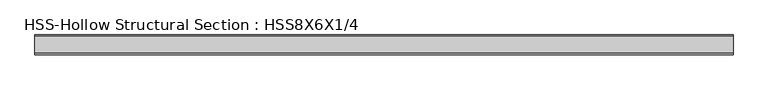
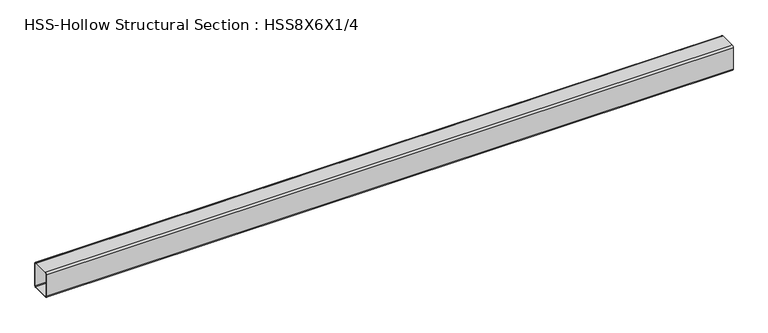
"""IFC4 building model written with IfcOpenShell, lengths in millimetres: beam geometry, HSS-Hollow Structural Section : HSS8X6X1/4."""

from ifc_helpers import new_model, si_unit, point, frame, frame_2d, origin, place, context, project, spatial, polyline, circle_curve, trimmed, segment, composite_curve, outline, extrude, source, transform, mapped, element, save


def hss_hollow_structural_section_hss8x6x1_4_86b5094b(model_context):
    return source(origin(), model_context, "Body", "SweptSolid", [
        extrude(outline(composite_curve([segment(trimmed(circle_curve(frame_2d((-64.3636, 89.7636)), 11.8364), [point((-76.2, 89.7636))], [point((-64.3636, 101.6))], False, "CARTESIAN"), True, "CONTINUOUS"), segment(polyline([(-64.3636, 101.6), (64.3636, 101.6)]), True, "CONTINUOUS"), segment(trimmed(circle_curve(frame_2d((64.3636, 89.7636)), 11.8364), [point((64.3636, 101.6))], [point((76.2, 89.7636))], False, "CARTESIAN"), True, "CONTINUOUS"), segment(polyline([(76.2, 89.7636), (76.2, -89.7636)]), True, "CONTINUOUS"), segment(trimmed(circle_curve(frame_2d((64.3636, -89.7636)), 11.8364), [point((76.2, -89.7636))], [point((64.3636, -101.6))], False, "CARTESIAN"), True, "CONTINUOUS"), segment(polyline([(64.3636, -101.6), (-64.3636, -101.6)]), True, "CONTINUOUS"), segment(trimmed(circle_curve(frame_2d((-64.3636, -89.7636)), 11.8364), [point((-64.3636, -101.6))], [point((-76.2, -89.7636))], False, "CARTESIAN"), True, "CONTINUOUS"), segment(polyline([(-76.2, -89.7636), (-76.2, 89.7636)]), True, "CONTINUOUS")], self_intersect=False), holes=[composite_curve([segment(polyline([(64.3636, 95.6818), (-64.3636, 95.6818)]), True, "CONTINUOUS"), segment(trimmed(circle_curve(frame_2d((-64.3636, 89.7636)), 5.9182), [point((-64.3636, 95.6818))], [point((-70.2818, 89.7636))], True, "CARTESIAN"), True, "CONTINUOUS"), segment(polyline([(-70.2818, 89.7636), (-70.2818, -89.7636)]), True, "CONTINUOUS"), segment(trimmed(circle_curve(frame_2d((-64.3636, -89.7636)), 5.9182), [point((-70.2818, -89.7636))], [point((-64.3636, -95.6818))], True, "CARTESIAN"), True, "CONTINUOUS"), segment(polyline([(-64.3636, -95.6818), (64.3636, -95.6818)]), True, "CONTINUOUS"), segment(trimmed(circle_curve(frame_2d((64.3636, -89.7636)), 5.9182), [point((64.3636, -95.6818))], [point((70.2818, -89.7636))], True, "CARTESIAN"), True, "CONTINUOUS"), segment(polyline([(70.2818, -89.7636), (70.2818, 89.7636)]), True, "CONTINUOUS"), segment(trimmed(circle_curve(frame_2d((64.3636, 89.7636)), 5.9182), [point((70.2818, 89.7636))], [point((64.3636, 95.6818))], True, "CARTESIAN"), True, "CONTINUOUS")], self_intersect=False)]), frame((-2667.0, 0.0, 0.0), z_axis=(1.0, 0.0, 0.0), x_axis=(0.0, 1.0, 0.0)), (0.0, 0.0, 1.0), 5334.0),
    ])


if __name__ == "__main__":
    model = new_model("IFC4")
    model_context = context("Model", 3, world=origin())
    ifc_project = project(units=[si_unit("LENGTHUNIT", "METRE", prefix="MILLI")], contexts=[model_context])
    site = spatial("IfcSite", under=ifc_project)
    building = spatial("IfcBuilding", under=site)
    placement = place(None, origin())
    hss_hollow_structural_section_hss8x6x1_4_shape = hss_hollow_structural_section_hss8x6x1_4_86b5094b(model_context)
    element("IfcBeam", 1, ObjectType="HSS-Hollow Structural Section : HSS8X6X1/4", at=placement, inside=building, context=model_context, shape_type="MappedRepresentation", body=[
        mapped(hss_hollow_structural_section_hss8x6x1_4_shape, transform((0.0, 0.0, 0.0), x_axis=(1.0, 0.0, 0.0), y_axis=(0.0, 1.0, 0.0), z_axis=(0.0, 0.0, 1.0))),
    ])
    save(model, "model.ifc")

# Revit data of these elements
# Type "HSS-Hollow Structural Section : HSS8X6X1/4"
#   Assembly Code = "B10"
#   Shape = "Rect."
#   W = 22.4
#   Ht = 0' - 8"
#   Length [instance default] = 5' - 0"
#   b = 0' - 6"
#   kr = 0' - 0.466"
#   t = 0' - 0.233"
#   A = 0.0428472 SF
#   Structural Material [instance default] = Steel ASTM A500, Grade B, Rectangular and Square
# Element 1 (IfcBeam, "HSS-Hollow Structural Section : HSS8X6X1/4")
#   Structural Material = TUBE STEEL INLINE WITH EXISTING X BRACING
#   Materials on its faces: "TUBE STEEL INLINE WITH EXISTING X BRACING"
# Materials
#   "Steel ASTM A500, Grade B, Rectangular and Square": class "Metal", colour RGB 199 199 199, transparency 0, Description = "Carbon steel", Cost = 0
#   "TUBE STEEL INLINE WITH EXISTING X BRACING": class "Generic", colour RGB 120 120 120, transparency 0, Cost = 0
